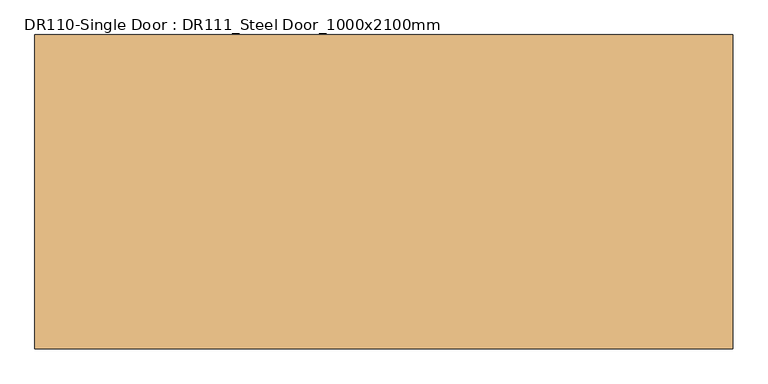
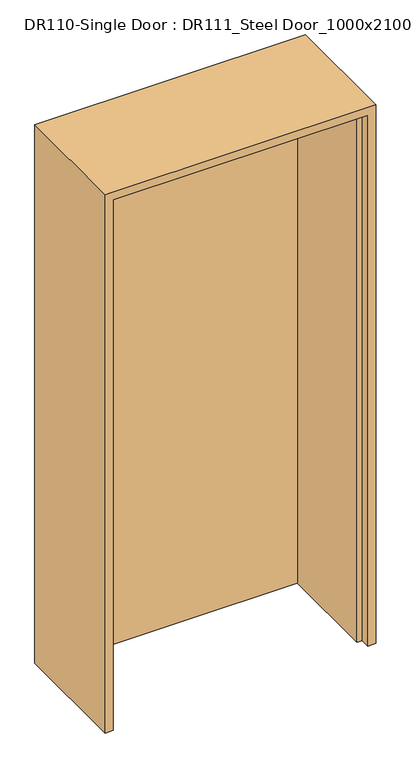
"""IFC4 building model written with IfcOpenShell, lengths in millimetres: door geometry, DR110-Single Door : DR111_Steel Door_1000x2100mm."""

from ifc_helpers import new_model, si_unit, origin, origin_with_axes, place, context, project, spatial, polyline, outline, extrude, faceted_brep, source, transform, mapped, element, save


def dr110_single_door_dr111_steel_door_1000x2100mm_e52ce95f(model_context):
    return source(origin(), model_context, "Body", "SolidModel", [
        extrude(outline(polyline([(470.0, 225.0), (470.0, 190.0), (-470.0, 190.0), (-470.0, 225.0), (470.0, 225.0)])), origin_with_axes(), (0.0, 0.0, 1.0), 2070.0),
        faceted_brep([(470.0, 225.0, 0.0), (500.0, 225.0, 0.0), (500.0, -225.0, 0.0), (470.0, -225.0, 0.0), (470.0, -190.0, 0.0), (450.0, -190.0, 0.0), (450.0, 190.0, 0.0), (470.0, 190.0, 0.0), (470.0, 225.0, 2070.0), (-470.0, 225.0, 2070.0), (-470.0, 225.0, 0.0), (-500.0, 225.0, 0.0), (-500.0, 225.0, 2100.0), (500.0, 225.0, 2100.0), (500.0, -225.0, 2100.0), (-500.0, -225.0, 2100.0), (-500.0, -225.0, 0.0), (-470.0, -225.0, 0.0), (-470.0, -225.0, 2070.0), (470.0, -225.0, 2070.0), (470.0, -190.0, 2070.0), (-470.0, -190.0, 2070.0), (-470.0, -190.0, 0.0), (-450.0, -190.0, 0.0), (-450.0, -190.0, 2050.0), (450.0, -190.0, 2050.0), (450.0, 190.0, 2050.0), (-450.0, 190.0, 2050.0), (-450.0, 190.0, 0.0), (-470.0, 190.0, 0.0), (-470.0, 190.0, 2070.0), (470.0, 190.0, 2070.0)], [[[0, 1, 2, 3, 4, 5, 6, 7]], [[1, 0, 8, 9, 10, 11, 12, 13]], [[2, 1, 13, 14]], [[3, 2, 14, 15, 16, 17, 18, 19]], [[4, 3, 19, 20]], [[5, 4, 20, 21, 22, 23, 24, 25]], [[6, 5, 25, 26]], [[7, 6, 26, 27, 28, 29, 30, 31]], [[0, 7, 31, 8]], [[9, 30, 29, 10]], [[10, 29, 28, 23, 22, 17, 16, 11]], [[15, 12, 11, 16]], [[21, 18, 17, 22]], [[27, 24, 23, 28]], [[14, 13, 12, 15]], [[20, 19, 18, 21]], [[26, 25, 24, 27]], [[8, 31, 30, 9]]]),
    ])


if __name__ == "__main__":
    model = new_model("IFC4")
    model_context = context("Model", 3, world=origin())
    ifc_project = project(units=[si_unit("LENGTHUNIT", "METRE", prefix="MILLI")], contexts=[model_context])
    site = spatial("IfcSite", under=ifc_project)
    building = spatial("IfcBuilding", under=site)
    placement = place(None, origin())
    dr110_single_door_dr111_steel_door_1000x2100mm_shape = dr110_single_door_dr111_steel_door_1000x2100mm_e52ce95f(model_context)
    element("IfcDoor", 1, ObjectType="DR110-Single Door : DR111_Steel Door_1000x2100mm", at=placement, inside=building, context=model_context, shape_type="MappedRepresentation", body=[
        mapped(dr110_single_door_dr111_steel_door_1000x2100mm_shape, transform((0.0, 0.0, 0.0), x_axis=(1.0, 0.0, 0.0), y_axis=(0.0, 1.0, 0.0), z_axis=(0.0, 0.0, 1.0))),
    ])
    save(model, "model.ifc")

# Revit data of these elements
# Type "DR110-Single Door : DR111_Steel Door_1000x2100mm"
#   Type Mark = "SD"
#   Analytic Construction = "<None>"
#   프레임 투영 외부. = 25 mm
#   프레임 투영 내부. = 25 mm
#   프레임 폭 = 75 mm
#   Height = 2100 mm
#   Width = 1000 mm
#   Define Thermal Properties by = 1
#   문 패널 = SD1 문 패널
#   문 프레임 = A04AQ098-00002_Steel Door_non FP_single
#   Function = (empty or 0)
#   Wall Closure = (empty or 0)
# Element 1 (IfcDoor, "DR110-Single Door : DR111_Steel Door_1000x2100mm")
#   Materials on its faces: "A04AQ098-00002_Steel Door_non FP_single", "SD1 문 패널"
# Materials
#   "SD1 문 패널": class "금속", colour RGB 247 247 247, transparency 0, Description = "STEEL DOOR (1000Wx2100H)"
#   "A04AQ098-00002_Steel Door_non FP_single": class "금속", colour RGB 247 247 247, transparency 0, Description = "Steel Door", W00) Work Master Code = "A04AQ098-00002", W01) Work Master_Lv1 = "Finishing Work", W02) Work Master_Lv2 = "Door & Window Work", W03) Work Master_Spec.1 = "Steel Door w/ Steel Frame", W04) Work Master_Spec.2 = "Fire Protective Rating: N/A, Single Door", W05) Work Master_Spec.3 = "w/ Hardware & Accessories", Cost = 0
